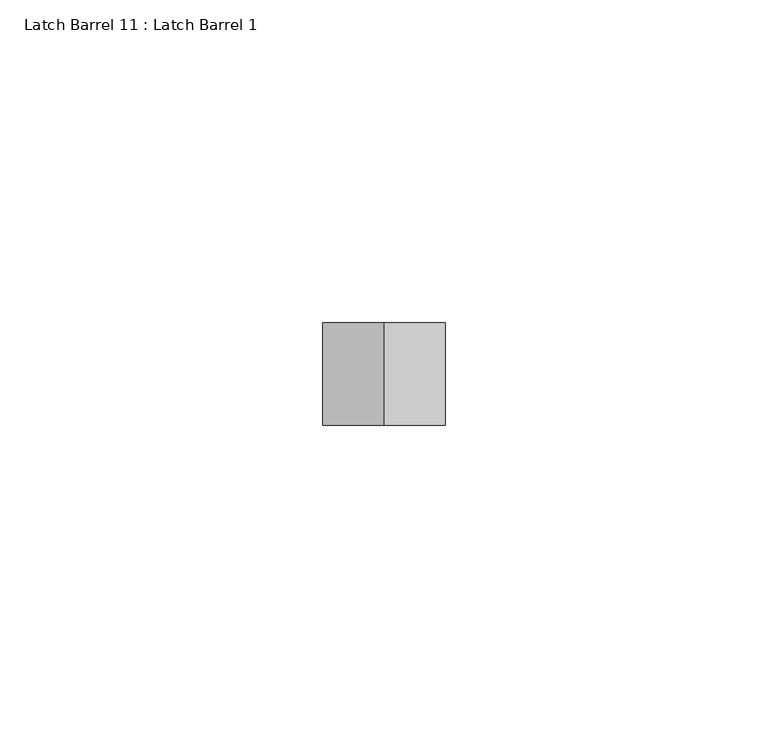
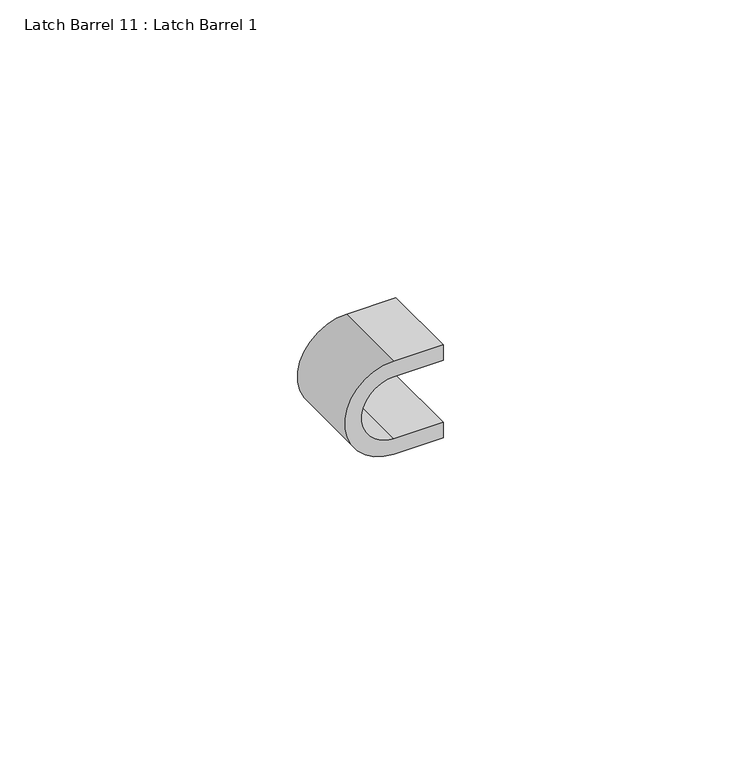
"""IFC4 building model written with IfcOpenShell, lengths in millimetres: proxy geometry, Latch Barrel 11 : Latch Barrel 1."""

from ifc_helpers import new_model, si_unit, point, frame, frame_2d, origin, place, context, project, spatial, polyline, circle_curve, trimmed, segment, composite_curve, outline, extrude, source, transform, mapped, element, save


def latch_barrel_11_latch_barrel_1_55035a22(model_context):
    return source(origin(), model_context, "Body", "SweptSolid", [
        extrude(outline(composite_curve([segment(trimmed(circle_curve(frame_2d((1066.8, 587312.7185739)), 6.35), [point((1060.45, 587312.7185739))], [point((1073.15, 587312.7185739))], True, "CARTESIAN"), True, "CONTINUOUS"), segment(polyline([(1073.15, 587312.7185739), (1073.15, 587322.2435739), (1076.325, 587322.2435739), (1076.325, 587312.7185739)]), True, "CONTINUOUS"), segment(trimmed(circle_curve(frame_2d((1066.8, 587312.7185739)), 9.525), [point((1076.325, 587312.7185739))], [point((1057.275, 587312.7185739))], False, "CARTESIAN"), True, "CONTINUOUS"), segment(polyline([(1057.275, 587312.7185739), (1057.275, 587322.2435739), (1060.45, 587322.2435739), (1060.45, 587312.7185739)]), True, "CONTINUOUS")], self_intersect=False)), frame((0.0, -532906.0413841, 0.0), z_axis=(0.0, 1.0, 0.0), x_axis=(0.0, 0.0, 1.0)), (0.0, 0.0, 1.0), 15.875),
    ])


if __name__ == "__main__":
    model = new_model("IFC4")
    model_context = context("Model", 3, world=origin())
    ifc_project = project(units=[si_unit("LENGTHUNIT", "METRE", prefix="MILLI")], contexts=[model_context])
    site = spatial("IfcSite", under=ifc_project)
    building = spatial("IfcBuilding", under=site)
    placement = place(None, origin())
    latch_barrel_11_latch_barrel_1_shape = latch_barrel_11_latch_barrel_1_55035a22(model_context)
    element("IfcBuildingElementProxy", 1, Name="Latch Barrel 11 : Latch Barrel 1", ObjectType="Latch Barrel 11 : Latch Barrel 1", at=placement, inside=building, context=model_context, shape_type="MappedRepresentation", body=[
        mapped(latch_barrel_11_latch_barrel_1_shape, transform((0.0, 0.0, 0.0), x_axis=(1.0, 0.0, 0.0), y_axis=(0.0, 1.0, 0.0), z_axis=(0.0, 0.0, 1.0))),
    ])
    save(model, "model.ifc")

# Revit data of these elements
# Element 1 (IfcBuildingElementProxy, "Latch Barrel 11 : Latch Barrel 1")
#   Materials on its faces: "GALV. GATE LATCH"
# Materials
#   "GALV. GATE LATCH": class "Metal", colour RGB 189 187 185, transparency 0, Description = "Carbon steel", Cost = 0
